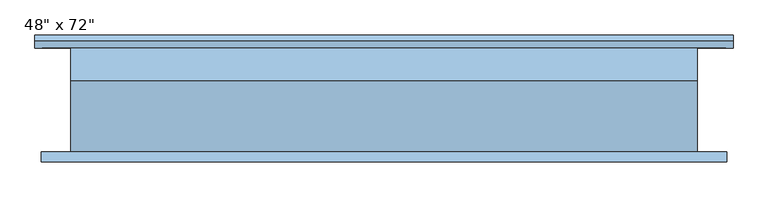
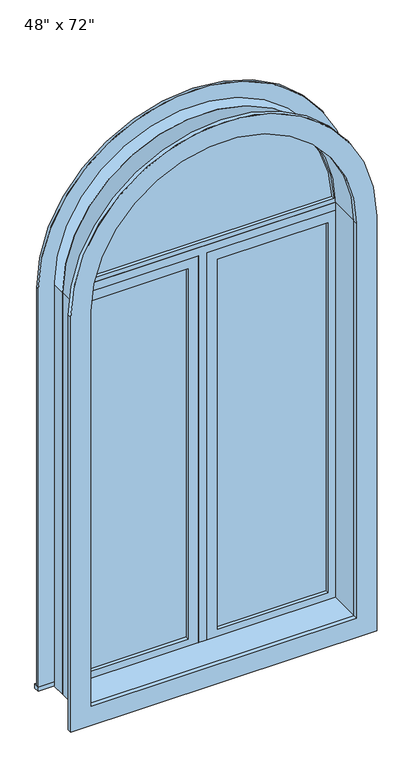
"""IFC4 building model written with IfcOpenShell, lengths in millimetres: window geometry."""

from ifc_helpers import new_model, si_unit, point, frame, frame_2d, origin, place, context, project, spatial, polyline, circle_curve, trimmed, segment, composite_curve, outline, extrude, source, transform, mapped, element, save


def window_5c2d0a27(model_context):
    return source(origin(), model_context, "Body", "SweptSolid", [
        extrude(outline(composite_curve([segment(polyline([(2152.65, -658.7478419), (247.65, -658.7478419), (247.65, 674.7521581), (2152.65, 674.7521581)]), True, "CONTINUOUS"), segment(trimmed(circle_curve(frame_2d((2152.65, 8.0021581)), 666.75), [point((2152.65, 674.7521581))], [point((2152.65, -658.7478419))], False, "CARTESIAN"), True, "CONTINUOUS")], self_intersect=False), holes=[composite_curve([segment(trimmed(circle_curve(frame_2d((2152.65, 8.0021581)), 577.85), [point((2152.65, -569.8478419))], [point((2152.65, 585.8521581))], True, "CARTESIAN"), True, "CONTINUOUS"), segment(polyline([(2152.65, 585.8521581), (336.55, 585.8521581), (336.55, -569.8478419), (2152.65, -569.8478419)]), True, "CONTINUOUS")], self_intersect=False)]), frame((0.0, -120.65, 0.0), z_axis=(0.0, 1.0, 0.0), x_axis=(0.0, 0.0, 1.0)), (0.0, 0.0, 1.0), 19.05),
        extrude(outline(composite_curve([segment(trimmed(circle_curve(frame_2d((2152.65, 8.0021581)), 571.5), [point((2171.6999995, 579.1845699))], [point((2171.6999995, -563.1802537))], False, "CARTESIAN"), True, "CONTINUOUS"), segment(polyline([(2171.6999995, -563.1802537), (2171.6999995, 579.1845699)]), True, "CONTINUOUS")], self_intersect=False)), frame((0.0, 53.975, 0.0), z_axis=(0.0, 1.0, 0.0), x_axis=(0.0, 0.0, 1.0)), (0.0, 0.0, 1.0), 12.7),
        extrude(outline(composite_curve([segment(trimmed(circle_curve(frame_2d((2152.65, 8.0021581)), 590.55), [point((2152.65, 598.5521581))], [point((2152.65, -582.5478419))], False, "CARTESIAN"), True, "CONTINUOUS"), segment(polyline([(2152.65, -582.5478419), (2152.65, 598.5521581)]), True, "CONTINUOUS")], self_intersect=False), holes=[composite_curve([segment(polyline([(2171.6999995, 579.1845698), (2171.6999995, -563.1802537)]), True, "CONTINUOUS"), segment(trimmed(circle_curve(frame_2d((2152.65, 8.0021581)), 571.5), [point((2171.6999995, -563.1802537))], [point((2171.6999995, 579.1845698))], True, "CARTESIAN"), True, "CONTINUOUS")], self_intersect=False)]), frame((0.0, 38.1, 0.0), z_axis=(0.0, 1.0, 0.0), x_axis=(0.0, 0.0, 1.0)), (0.0, 0.0, 1.0), 44.45),
        extrude(outline(composite_curve([segment(polyline([(304.8, -601.5978419), (304.8, 617.6021581), (2152.65, 617.6021581)]), True, "CONTINUOUS"), segment(trimmed(circle_curve(frame_2d((2152.65, 8.0021581)), 609.6), [point((2152.65, 617.6021581))], [point((2152.65, -601.5978419))], False, "CARTESIAN"), True, "CONTINUOUS"), segment(polyline([(2152.65, -601.5978419), (304.8, -601.5978419)]), True, "CONTINUOUS")], self_intersect=False), holes=[composite_curve([segment(polyline([(323.85, -582.5478419), (2152.65, -582.5478419)]), True, "CONTINUOUS"), segment(trimmed(circle_curve(frame_2d((2152.65, 8.0021581)), 590.55), [point((2152.65, -582.5478419))], [point((2152.65, 598.5521581))], True, "CARTESIAN"), True, "CONTINUOUS"), segment(polyline([(2152.65, 598.5521581), (323.85, 598.5521581), (323.85, -582.5478419)]), True, "CONTINUOUS")], self_intersect=False)]), frame((0.0, 38.1, 0.0), z_axis=(0.0, 1.0, 0.0), x_axis=(0.0, 0.0, 1.0)), (0.0, 0.0, 1.0), 63.5),
        extrude(outline(polyline([(71.5021581, 66.675), (554.1021581, 66.675), (554.1021581, 53.975), (71.5021581, 53.975), (71.5021581, 66.675)])), frame((0.0, 0.0, 368.3), z_axis=(0.0, 0.0, 1.0), x_axis=(1.0, 0.0, 0.0)), (0.0, 0.0, 1.0), 1701.8),
        extrude(outline(polyline([(2114.55, 27.0521581), (323.85, 27.0521581), (323.85, 598.5521581), (2114.55, 598.5521581), (2114.55, 27.0521581)]), holes=[polyline([(2070.1, 71.5021581), (2070.1, 554.1021581), (368.3, 554.1021581), (368.3, 71.5021581), (2070.1, 71.5021581)])]), frame((0.0, 38.1, 0.0), z_axis=(0.0, 1.0, 0.0), x_axis=(0.0, 0.0, 1.0)), (0.0, 0.0, 1.0), 44.45),
        extrude(outline(polyline([(323.85, -11.0478419), (323.85, 27.0521581), (2114.55, 27.0521581), (2114.55, 598.5521581), (2152.65, 598.5521581), (2152.65, -582.5478419), (2114.55, -582.5478419), (2114.55, -11.0478419), (323.85, -11.0478419)])), frame((0.0, 38.1, 0.0), z_axis=(0.0, 1.0, 0.0), x_axis=(0.0, 0.0, 1.0)), (0.0, 0.0, 1.0), 63.5),
        extrude(outline(polyline([(-671.4478419, 127.0), (687.4521581, 127.0), (687.4521581, 101.6), (-671.4478419, 101.6), (-671.4478419, 127.0)])), frame((0.0, 0.0, 304.8), z_axis=(0.0, 0.0, 1.0), x_axis=(1.0, 0.0, 0.0)), (0.0, 0.0, 1.0), 19.05),
        extrude(outline(composite_curve([segment(polyline([(323.85, 598.5521581), (323.85, 687.4521581), (2152.65, 687.4521581)]), True, "CONTINUOUS"), segment(trimmed(circle_curve(frame_2d((2152.65, 8.0021581)), 679.45), [point((2152.65, 687.4521581))], [point((2152.65, -671.4478419))], False, "CARTESIAN"), True, "CONTINUOUS"), segment(polyline([(2152.65, -671.4478419), (323.85, -671.4478419), (323.85, -582.5478419), (2152.65, -582.5478419)]), True, "CONTINUOUS"), segment(trimmed(circle_curve(frame_2d((2152.65, 8.0021581)), 590.55), [point((2152.65, -582.5478419))], [point((2152.65, 598.5521581))], True, "CARTESIAN"), True, "CONTINUOUS"), segment(polyline([(2152.65, 598.5521581), (323.85, 598.5521581)]), True, "CONTINUOUS")], self_intersect=False)), frame((0.0, 101.6, 0.0), z_axis=(0.0, 1.0, 0.0), x_axis=(0.0, 0.0, 1.0)), (0.0, 0.0, 1.0), 12.7),
        extrude(outline(polyline([(-55.4978419, 53.975), (-538.0978419, 53.975), (-538.0978419, 66.675), (-55.4978419, 66.675), (-55.4978419, 53.975)])), frame((0.0, 0.0, 368.3), z_axis=(0.0, 0.0, 1.0), x_axis=(1.0, 0.0, 0.0)), (0.0, 0.0, 1.0), 1701.8),
        extrude(outline(polyline([(2114.55, -582.5478419), (323.85, -582.5478419), (323.85, -11.0478419), (2114.55, -11.0478419), (2114.55, -582.5478419)]), holes=[polyline([(2070.1, -538.0978419), (2070.1, -55.4978419), (368.3, -55.4978419), (368.3, -538.0978419), (2070.1, -538.0978419)])]), frame((0.0, 38.1, 0.0), z_axis=(0.0, 1.0, 0.0), x_axis=(0.0, 0.0, 1.0)), (0.0, 0.0, 1.0), 44.45),
        extrude(outline(composite_curve([segment(polyline([(304.8, 617.6021581), (2152.65, 617.6021581)]), True, "CONTINUOUS"), segment(trimmed(circle_curve(frame_2d((2152.65, 8.0021581)), 609.6), [point((2152.65, 617.6021581))], [point((2152.65, -601.5978419))], False, "CARTESIAN"), True, "CONTINUOUS"), segment(polyline([(2152.65, -601.5978419), (304.8, -601.5978419), (304.8, 617.6021581)]), True, "CONTINUOUS")], self_intersect=False), holes=[composite_curve([segment(polyline([(336.55, 585.8521581), (336.55, -569.8478419), (2152.65, -569.8478419)]), True, "CONTINUOUS"), segment(trimmed(circle_curve(frame_2d((2152.65, 8.0021581)), 577.85), [point((2152.65, -569.8478419))], [point((2152.65, 585.8521581))], True, "CARTESIAN"), True, "CONTINUOUS"), segment(polyline([(2152.65, 585.8521581), (336.55, 585.8521581)]), True, "CONTINUOUS")], self_intersect=False)]), frame((0.0, -101.6, 0.0), z_axis=(0.0, 1.0, 0.0), x_axis=(0.0, 0.0, 1.0)), (0.0, 0.0, 1.0), 139.7),
    ])


if __name__ == "__main__":
    model = new_model("IFC4")
    model_context = context("Model", 3, world=origin())
    ifc_project = project(units=[si_unit("LENGTHUNIT", "METRE", prefix="MILLI")], contexts=[model_context])
    site = spatial("IfcSite", under=ifc_project)
    building = spatial("IfcBuilding", under=site)
    placement = place(None, origin())
    window_shape = window_5c2d0a27(model_context)
    element("IfcWindow", 1, ObjectType="Combination Rtp with Trim : 48\" x 72\"", at=placement, inside=building, context=model_context, shape_type="MappedRepresentation", body=[
        mapped(window_shape, transform((0.0, 0.0, 0.0), x_axis=(1.0, 0.0, 0.0), y_axis=(0.0, 1.0, 0.0), z_axis=(0.0, 0.0, 1.0))),
    ])
    save(model, "model.ifc")

# Revit data of these elements
# Type "Combination Rtp with Trim : 48\" x 72\""
#   Type Mark = "25"
#   Construction Type Id = "SGL"
#   Assembly Code = "B2020100"
#   Analytic Construction = "Large single-glazed windows"
#   Visual Light Transmittance = 0.9
#   Solar Heat Gain Coefficient = 0.86
#   Heat Transfer Coefficient (U) = 5.5617 W/(m²·K)
#   Height = 6' - 0"
#   Default Sill Height = 1' - 0"
#   Trim Projection - Ext. = 0' - 0 1/2"
#   Trim Projection - Int. = 0' - 0 3/4"
#   Trim Width - Exterior = 0' - 3 1/2"
#   Trim Width - Interior = 0' - 3 1/2"
#   Width = 4' - 0"
#   Window Inset = 0' - 0 3/4"
#   Glass Pane Material = Glass
#   Sash Material = Sash
#   Trim Exterior Material = Trim
#   Trim Interior Material = Trim
#   Wall Closure = (empty or 0)
# Element 1 (IfcWindow, "Combination Rtp with Trim : 48\" x 72\"")
#   Materials on its faces: "Sash", "Trim", "Glass"
# Materials
#   "Glass": class "Glass", colour RGB 0 128 192, transparency 0.75, Description = "Soda Lime Glass", Cost = 0
#   "Sash": class "Wood", colour RGB 224 178 126, transparency 0, Cost = 0
#   "Trim": class "Wood", colour RGB 224 178 126, transparency 0
